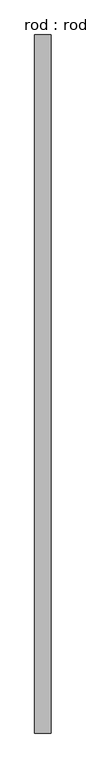
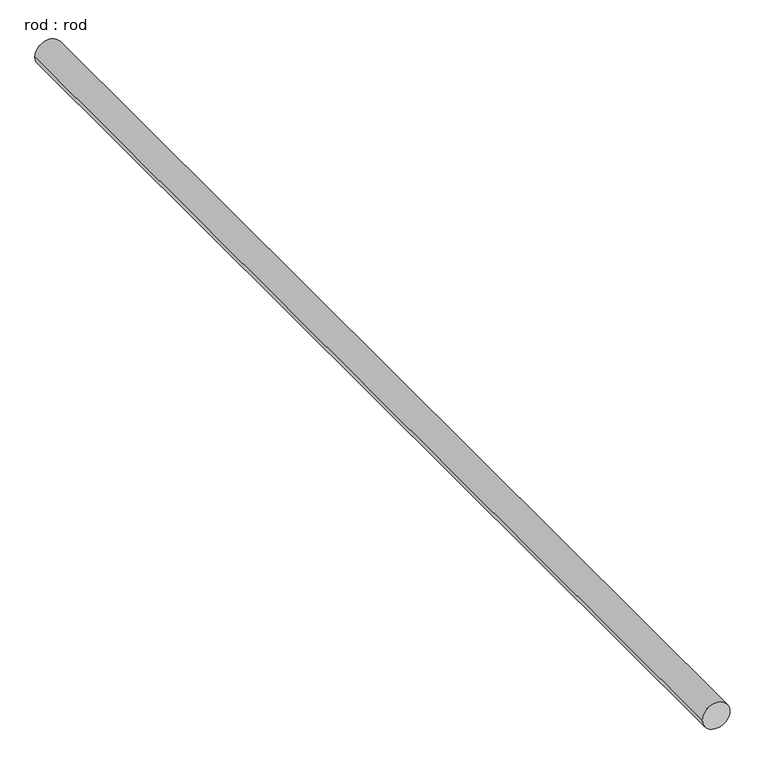
"""IFC4 building model written with IfcOpenShell, lengths in millimetres: proxy geometry, rod : rod."""

from ifc_helpers import new_model, si_unit, point, frame, frame_2d, origin, place, context, project, spatial, circle_curve, trimmed, segment, composite_curve, outline, extrude, source, transform, mapped, element, save


def rod_rod_e40903e6(model_context):
    return source(origin(), model_context, "Body", "SweptSolid", [
        extrude(outline(composite_curve([segment(trimmed(circle_curve(frame_2d((0.0108462, 0.0)), 200.0), [point((0.0108462, 200.0))], [point((0.0108462, -200.0))], False, "CARTESIAN"), True, "CONTINUOUS"), segment(trimmed(circle_curve(frame_2d((0.0108462, 0.0)), 200.0), [point((0.0108462, -200.0))], [point((0.0108462, 200.0))], False, "CARTESIAN"), True, "CONTINUOUS")], self_intersect=False)), frame((0.0, -4325.341033, 0.0), z_axis=(0.0, 1.0, 0.0), x_axis=(0.0, 0.0, 1.0)), (0.0, 0.0, 1.0), 16836.1392968),
    ])


if __name__ == "__main__":
    model = new_model("IFC4")
    model_context = context("Model", 3, world=origin())
    ifc_project = project(units=[si_unit("LENGTHUNIT", "METRE", prefix="MILLI")], contexts=[model_context])
    site = spatial("IfcSite", under=ifc_project)
    building = spatial("IfcBuilding", under=site)
    placement = place(None, origin())
    rod_rod_shape = rod_rod_e40903e6(model_context)
    element("IfcBuildingElementProxy", 1, Name="rod : rod", ObjectType="rod : rod", at=placement, inside=building, context=model_context, shape_type="MappedRepresentation", body=[
        mapped(rod_rod_shape, transform((0.0, 0.0, 0.0), x_axis=(1.0, 0.0, 0.0), y_axis=(0.0, 1.0, 0.0), z_axis=(0.0, 0.0, 1.0))),
    ])
    save(model, "model.ifc")

# Revit data of these elements
# Type "rod : rod"
#   Default Elevation = 0
